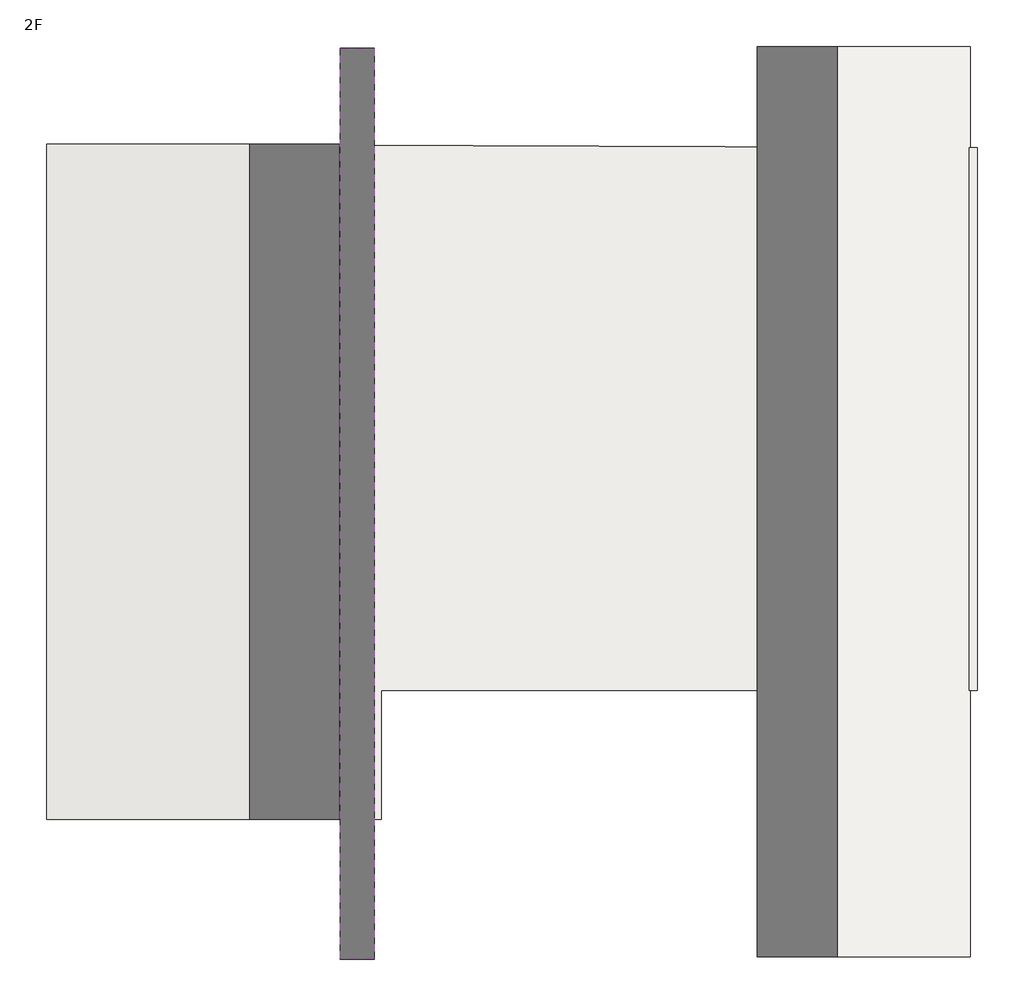
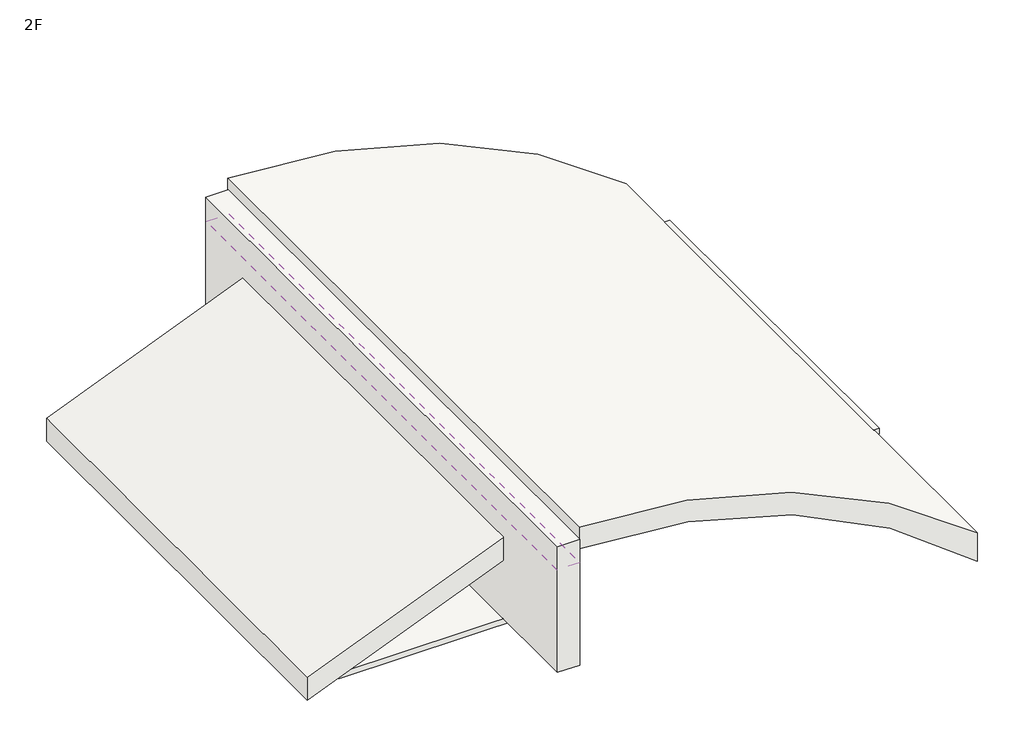
# One storey: 5 roofs.
"""IFC4 building model written with IfcOpenShell, lengths in millimetres."""

from ifc_helpers import new_model, si_unit, point, frame, frame_2d, origin, place, context, project, spatial, polyline, circle_curve, trimmed, segment, composite_curve, outline, extrude, element, save

model = new_model("IFC4")

# Units and contexts
model_context = context("Model", 3, world=origin())
ifc_project = project(units=[si_unit("LENGTHUNIT", "METRE", prefix="MILLI")], contexts=[model_context])

# Site, building, storey
site = spatial("IfcSite", under=ifc_project)
building = spatial("IfcBuilding", under=site)
storey = spatial("IfcBuildingStorey", under=building, Name="2F", Elevation=6450.0)

# Roofs
placement = place(None, origin())
element("IfcRoof", 1, ObjectType="Generic - 400mm", at=placement, inside=storey, context=model_context, shape_type="SweptSolid", body=[
    extrude(outline(composite_curve([segment(polyline([(9109.5004401, -15760.6826666), (8709.4956906, -15760.6826666)]), True, "CONTINUOUS"), segment(trimmed(circle_curve(frame_2d((-1731.4641647, -15708.8367035)), 10441.0885784), [point((8709.4956906, -15760.6826666))], [point((6008.1810273, -8700.6826666))], True, "CARTESIAN"), True, "CONTINUOUS"), segment(polyline([(6008.1810273, -8700.6826666), (6539.8705862, -8700.6826666)]), True, "CONTINUOUS"), segment(trimmed(circle_curve(frame_2d((-1731.4641647, -15708.8367035)), 10841.0885784), [point((6539.8705862, -8700.6826666))], [point((9109.5004401, -15760.6826666))], False, "CARTESIAN"), True, "CONTINUOUS")], self_intersect=False)), frame((0.0, -1720.1288648, 0.0), z_axis=(0.0, 1.0, 0.0), x_axis=(0.0, 0.0, 1.0)), (0.0, 0.0, 1.0), 10782.5655583),
])
element("IfcRoof", 2, ObjectType="Generic - 400mm", at=placement, inside=storey, context=model_context, shape_type="SweptSolid", body=[
    extrude(outline(polyline([(-15760.6826666, -1747.8561761), (-16160.6826666, -1747.8561761), (-16160.6826666, 9042.8723436), (-15760.6826666, 9042.8723436), (-15760.6826666, -1747.8561761)])), frame((0.0, 0.0, 6550.0), z_axis=(0.0, 0.0, 1.0), x_axis=(1.0, 0.0, 0.0)), (0.0, 0.0, 1.0), 2359.4980653),
])
element("IfcRoof", 3, ObjectType="Generic - 400mm", at=placement, inside=storey, context=model_context, shape_type="SweptSolid", body=[
    extrude(outline(polyline([(8909.4980653, -16160.6826666), (8462.2834078, -16160.6826666), (8662.2857825, -15760.6826666), (9109.5004401, -15760.6826666), (8909.4980653, -16160.6826666)])), frame((0.0, -1740.2443602, 0.0), z_axis=(0.0, 1.0, 0.0), x_axis=(0.0, 0.0, 1.0)), (0.0, 0.0, 1.0), 10776.1228455),
])
element("IfcRoof", 4, ObjectType="Generic - 400mm", at=placement, inside=storey, context=model_context, shape_type="SweptSolid", body=[
    extrude(outline(polyline([(6680.6161776, -19639.4433339), (6249.2022805, -19639.4433339), (7672.7073355, -16116.1446865), (8104.1212326, -16116.1446865), (6680.6161776, -19639.4433339)])), frame((0.0, -94.9933886, 0.0), z_axis=(0.0, 1.0, 0.0), x_axis=(0.0, 0.0, 1.0)), (0.0, 0.0, 1.0), 8000.0),
])
element("IfcRoof", 5, ObjectType="roof", at=placement, inside=storey, context=model_context, shape_type="SweptSolid", body=[
    extrude(outline(polyline([(-19076.5903863, -94.9933886), (-19076.5903863, 7905.0066114), (-8616.5903863, 7865.0066114), (-8616.5903863, 1435.0066114), (-15676.5903863, 1435.0066114), (-15676.5903863, -94.9933886), (-19076.5903863, -94.9933886)])), frame((0.0, 0.0, 6450.0), z_axis=(0.0, 0.0, 1.0), x_axis=(1.0, 0.0, 0.0)), (0.0, 0.0, 1.0), 100.0),
])

save(model, "model.ifc")

# Revit data of these elements
# Project information
#   Project Issue Date = "Issue Date"
#   Project Status = "Project Status"
#   Client Name = "Owner"
#   Project Address = "Enter address here"
#   Project Name = "Project Name"
#   Project Number = "0001"
# Type "Generic - 400mm"
#   Layers, outside or top first: 40 cm no material (function 1)
# Type "roof"
#   Layers, outside or top first: 10 cm no material (function 1)
# Elements 1, 3 (IfcRoof, "Generic - 400mm")
#   built-in parameter 1001710 = 33615
#   Phase Created = New Construction
#   Materials on its faces: "Default Roof", "Brick, Common"
# Element 2 (IfcRoof, "Generic - 400mm")
#   built-in parameter 1001710 = 33615
#   Phase Created = New Construction
#   Materials on its faces: "Brick, Common", "Default Roof"
# Element 4 (IfcRoof, "Generic - 400mm")
#   built-in parameter 1001710 = 33615
#   Phase Created = New Construction
#   Materials on its faces: "Default Roof", "Brick, Common", "Parking Stripe"
# Element 5 (IfcRoof, "roof")
#   built-in parameter 1001705 = 21.4895 (stored number, unit not read)
#   built-in parameter 1001710 = 33615
#   Phase Created = New Construction
#   Materials on its faces: "Default Roof", "Earth", "Brick, Common"
# Materials
#   "Default Roof": class "Miscellaneous", colour RGB 0 127 0, transparency 0, Cost = 0
#   "Brick, Common": class "Masonry", colour RGB 170 100 105, transparency 0, Description = "Common brick", Cost = 0
#   "Parking Stripe": class "Paint", colour RGB 250 250 91, transparency 0, Cost = 0
#   "Earth": class "Generic", colour RGB 97 75 62, transparency 0, Description = "Soil", Cost = 0
